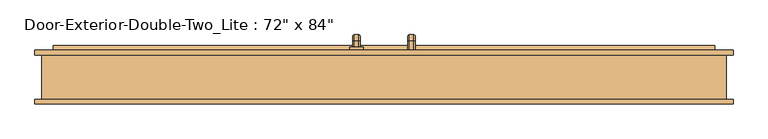
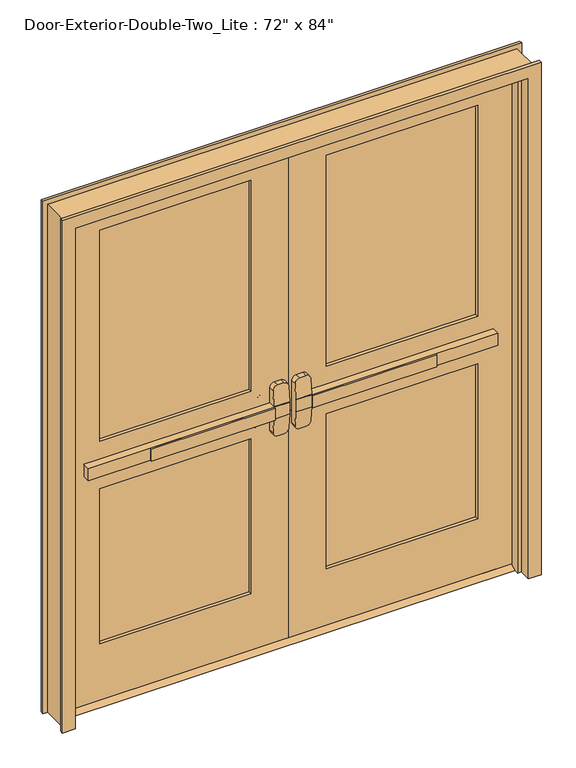
"""IFC4 building model written with IfcOpenShell, lengths in millimetres: door geometry."""

from ifc_helpers import new_model, si_unit, point, frame, frame_2d, origin, place, context, project, spatial, polyline, circle_curve, ellipse_curve, trimmed, segment, composite_curve, outline, extrude, faceted_brep, source, transform, mapped, element, save
from ifc_brep_helpers import plane_surface, cylinder_surface, revolved_surface, advanced_brep


def door_1ff579ad(model_context):
    return source(origin(), model_context, "Body", "SolidModel", [
        extrude(outline(polyline([(-575.7333333, -14.2875), (-575.7333333, -7.9375), (-76.2, -7.9375), (-76.2, -14.2875), (-575.7333333, -14.2875)])), frame((0.0, 0.0, 990.6), z_axis=(0.0, 0.0, 1.0), x_axis=(1.0, 0.0, 0.0)), (0.0, 0.0, 1.0), 50.8),
        advanced_brep(
        [(-12.7, -7.9375, 1041.4), (-76.2, -7.9375, 1041.4), (-825.5, -7.9375, 1041.4), (-825.5, -7.9375, 990.6), (-76.2, -7.9375, 990.6), (-12.7, -7.9375, 990.6), (-825.5, 23.8125, 1041.4), (-76.2, 23.8125, 1041.4), (-76.2, 23.8125, 1104.9), (-57.15, 23.8125, 1123.95), (-31.75, 23.8125, 1123.95), (-12.7, 23.8125, 1104.9), (-12.7, 23.8125, 927.1), (-31.75, 23.8125, 908.05), (-57.15, 23.8125, 908.05), (-76.2, 23.8125, 927.1), (-76.2, 23.8125, 990.6), (-825.5, 23.8125, 990.6), (-12.7, -4.7622533, 1041.4), (-76.2, -4.7622533, 1041.4), (-12.7, -4.7622533, 990.6), (-12.7, 0.2479269, 927.1), (-12.7, 0.2479269, 1104.9), (-76.2, -4.7622533, 990.6), (-76.2, 0.2479269, 1104.9), (-76.2, 0.2479269, 927.1), (-57.15, 1.750981, 1123.95), (-31.75, 1.750981, 1123.95), (-31.75, 1.750981, 908.05), (-57.15, 1.750981, 908.05)],
        [
            (0, 1),
            (1, 2),
            (2, 3),
            (3, 4),
            (4, 5),
            (5, 0),
            (6, 7),
            (7, 8),
            (8, 9, circle_curve(frame((-57.15, 23.8125, 1104.9), z_axis=(0.0, 1.0, 0.0), x_axis=(-1.0, 0.0, 0.0)), 19.05)),
            (9, 10),
            (10, 11, circle_curve(frame((-31.75, 23.8125, 1104.9), z_axis=(0.0, 1.0, 0.0), x_axis=(-1.0, 0.0, 0.0)), 19.05)),
            (11, 12),
            (12, 13, circle_curve(frame((-31.75, 23.8125, 927.1), z_axis=(0.0, 1.0, 0.0), x_axis=(-1.0, 0.0, 0.0)), 19.05)),
            (13, 14),
            (14, 15, circle_curve(frame((-57.15, 23.8125, 927.1), z_axis=(0.0, 1.0, 0.0), x_axis=(-1.0, 0.0, 0.0)), 19.05)),
            (15, 16),
            (16, 17),
            (17, 6),
            (0, 18),
            (18, 19),
            (19, 7),
            (6, 2),
            (5, 20),
            (20, 21),
            (21, 12),
            (11, 22),
            (22, 18),
            (16, 23),
            (23, 20),
            (3, 17),
            (19, 24),
            (24, 8),
            (15, 25),
            (25, 23),
            (9, 26),
            (26, 27),
            (27, 10),
            (13, 28),
            (28, 29),
            (29, 14),
            (29, 25, ellipse_curve(frame((-57.15, 0.2479269, 927.1), z_axis=(0.0, 0.9969018152893365, 0.07865602756830282), x_axis=(0.0, -0.07865602756830208, 0.9969018152893365)), 19.1092038, 19.05)),
            (24, 26, ellipse_curve(frame((-57.15, 0.2479269, 1104.9), z_axis=(0.0, 0.9969018152893376, -0.07865602756828934), x_axis=(0.0, -0.078656027568288, -0.9969018152893377)), 19.1092038, 19.05)),
            (27, 22, ellipse_curve(frame((-31.75, 0.2479269, 1104.9), z_axis=(0.0, 0.9969018152893376, -0.07865602756828934), x_axis=(0.0, -0.078656027568288, -0.9969018152893377)), 19.1092038, 19.05)),
            (21, 28, ellipse_curve(frame((-31.75, 0.2479269, 927.1), z_axis=(0.0, 0.9969018152893365, 0.07865602756830282), x_axis=(0.0, -0.07865602756830208, 0.9969018152893365)), 19.1092038, 19.05)),
        ],
        [
            plane_surface(frame((-12.7, -7.9375, 1041.4), z_axis=(0.0, -1.0, 0.0), x_axis=(1.0, 0.0, 0.0))),
            plane_surface(frame((-12.7, 23.8125, 1041.4), z_axis=(0.0, 1.0, 0.0), x_axis=(-1.0, 0.0, 0.0))),
            plane_surface(frame((-825.5, -7.9375, 1041.4), z_axis=(0.0, 0.0, 1.0), x_axis=(0.0, 1.0, 0.0))),
            plane_surface(frame((-12.7, -7.9375, 1041.4), z_axis=(1.0, 0.0, 0.0), x_axis=(0.0, 1.0, 0.0))),
            plane_surface(frame((-12.7, -7.9375, 990.6), z_axis=(0.0, 0.0, -1.0), x_axis=(0.0, 1.0, 0.0))),
            plane_surface(frame((-825.5, -7.9375, 990.6), z_axis=(-1.0, 0.0, 0.0), x_axis=(0.0, 1.0, 0.0))),
            plane_surface(frame((-76.2, -4.7622533, 927.1), z_axis=(-1.0, 0.0, 0.0), x_axis=(0.0, 1.0, 0.0))),
            plane_surface(frame((-57.15, -4.7622533, 1123.95), z_axis=(0.0, 0.0, 1.0), x_axis=(0.0, 1.0, 0.0))),
            plane_surface(frame((-31.75, -4.7622533, 908.05), z_axis=(0.0, 0.0, -1.0), x_axis=(0.0, 1.0, 0.0))),
            cylinder_surface(frame((-57.15, 23.8125, 927.1), z_axis=(0.0, -1.0, 0.0), x_axis=(-1.0, 0.0, 0.0)), 19.05),
            cylinder_surface(frame((-57.15, 23.8125, 1104.9), z_axis=(0.0, -1.0, 0.0), x_axis=(-1.0, 0.0, 0.0)), 19.05),
            cylinder_surface(frame((-31.75, 23.8125, 1104.9), z_axis=(0.0, -1.0, 0.0), x_axis=(-1.0, 0.0, 0.0)), 19.05),
            cylinder_surface(frame((-31.75, 23.8125, 927.1), z_axis=(0.0, -1.0, 0.0), x_axis=(-1.0, 0.0, 0.0)), 19.05),
            plane_surface(frame((-76.2, -4.7622533, 1041.4), z_axis=(0.0, -0.9969018152893376, 0.07865602756828934), x_axis=(1.0, 0.0, 0.0))),
            plane_surface(frame((-76.2, 1.750981, 908.05), z_axis=(0.0, -0.9969018152893365, -0.07865602756830282), x_axis=(1.0, 0.0, 0.0))),
        ],
        [
            (0, [[1, 2, 3, 4, 5, 6]]),
            (1, [[7, 8, 9, 10, 11, 12, 13, 14, 15, 16, 17, 18]]),
            (2, [[-2, -1, 19, 20, 21, -7, 22]]),
            (3, [[23, 24, 25, -12, 26, 27, -19, -6]]),
            (4, [[-17, 28, 29, -23, -5, -4, 30]]),
            (5, [[-22, -18, -30, -3]]),
            (6, [[-21, 31, 32, -8]]),
            (6, [[33, 34, -28, -16]]),
            (7, [[35, 36, 37, -10]]),
            (8, [[38, 39, 40, -14]]),
            (9, [[-40, 41, -33, -15]]),
            (10, [[-32, 42, -35, -9]]),
            (11, [[-37, 43, -26, -11]]),
            (12, [[-25, 44, -38, -13]]),
            (13, [[-27, -43, -36, -42, -31, -20]]),
            (14, [[-29, -34, -41, -39, -44, -24]]),
        ],
    ),
        extrude(outline(polyline([(68.2625, 12.7), (93.6625, 0.0), (-1.5875, 0.0), (23.8125, 12.7), (68.2625, 12.7)])), frame((-914.4, 0.0, 0.0), z_axis=(1.0, 0.0, 0.0), x_axis=(0.0, 1.0, 0.0)), (0.0, 0.0, 1.0), 1828.8),
        extrude(outline(polyline([(575.7333333, -14.2875), (76.2, -14.2875), (76.2, -7.9375), (575.7333333, -7.9375), (575.7333333, -14.2875)])), frame((0.0, 0.0, 990.6), z_axis=(0.0, 0.0, 1.0), x_axis=(1.0, 0.0, 0.0)), (0.0, 0.0, 1.0), 50.8),
        advanced_brep(
        [(12.7, -7.9375, 1041.4), (12.7, -7.9375, 990.6), (76.2, -7.9375, 990.6), (825.5, -7.9375, 990.6), (825.5, -7.9375, 1041.4), (76.2, -7.9375, 1041.4), (825.5, 23.8125, 1041.4), (825.5, 23.8125, 990.6), (76.2, 23.8125, 990.6), (76.2, 23.8125, 927.1), (57.15, 23.8125, 908.05), (31.75, 23.8125, 908.05), (12.7, 23.8125, 927.1), (12.7, 23.8125, 1104.9), (31.75, 23.8125, 1123.95), (57.15, 23.8125, 1123.95), (76.2, 23.8125, 1104.9), (76.2, 23.8125, 1041.4), (76.2, -4.7622533, 1041.4), (12.7, -4.7622533, 1041.4), (12.7, 0.2479269, 1104.9), (12.7, 0.2479269, 927.1), (12.7, -4.7622533, 990.6), (76.2, -4.7622533, 990.6), (76.2, 0.2479269, 927.1), (76.2, 0.2479269, 1104.9), (31.75, 1.750981, 1123.95), (57.15, 1.750981, 1123.95), (57.15, 1.750981, 908.05), (31.75, 1.750981, 908.05)],
        [
            (0, 1),
            (1, 2),
            (2, 3),
            (3, 4),
            (4, 5),
            (5, 0),
            (6, 7),
            (7, 8),
            (8, 9),
            (9, 10, circle_curve(frame((57.15, 23.8125, 927.1), z_axis=(0.0, 1.0, 0.0), x_axis=(1.0, 0.0, 0.0)), 19.05)),
            (10, 11),
            (11, 12, circle_curve(frame((31.75, 23.8125, 927.1), z_axis=(0.0, 1.0, 0.0), x_axis=(1.0, 0.0, 0.0)), 19.05)),
            (12, 13),
            (13, 14, circle_curve(frame((31.75, 23.8125, 1104.9), z_axis=(0.0, 1.0, 0.0), x_axis=(1.0, 0.0, 0.0)), 19.05)),
            (14, 15),
            (15, 16, circle_curve(frame((57.15, 23.8125, 1104.9), z_axis=(0.0, 1.0, 0.0), x_axis=(1.0, 0.0, 0.0)), 19.05)),
            (16, 17),
            (17, 6),
            (4, 6),
            (17, 18),
            (18, 19),
            (19, 0),
            (19, 20),
            (20, 13),
            (12, 21),
            (21, 22),
            (22, 1),
            (7, 3),
            (22, 23),
            (23, 8),
            (23, 24),
            (24, 9),
            (16, 25),
            (25, 18),
            (14, 26),
            (26, 27),
            (27, 15),
            (10, 28),
            (28, 29),
            (29, 11),
            (24, 28, ellipse_curve(frame((57.15, 0.2479269, 927.1), z_axis=(0.0, 0.9969018152893365, 0.07865602756830282), x_axis=(0.0, -0.07865602756830208, 0.9969018152893365)), 19.1092038, 19.05)),
            (27, 25, ellipse_curve(frame((57.15, 0.2479269, 1104.9), z_axis=(0.0, 0.9969018152893376, -0.07865602756828934), x_axis=(0.0, -0.078656027568288, -0.9969018152893377)), 19.1092038, 19.05)),
            (20, 26, ellipse_curve(frame((31.75, 0.2479269, 1104.9), z_axis=(0.0, 0.9969018152893376, -0.07865602756828934), x_axis=(0.0, -0.078656027568288, -0.9969018152893377)), 19.1092038, 19.05)),
            (29, 21, ellipse_curve(frame((31.75, 0.2479269, 927.1), z_axis=(0.0, 0.9969018152893365, 0.07865602756830282), x_axis=(0.0, -0.07865602756830208, 0.9969018152893365)), 19.1092038, 19.05)),
        ],
        [
            plane_surface(frame((12.7, -7.9375, 1041.4), z_axis=(0.0, -1.0, 0.0), x_axis=(-1.0, 0.0, 0.0))),
            plane_surface(frame((12.7, 23.8125, 1041.4), z_axis=(0.0, 1.0, 0.0), x_axis=(1.0, 0.0, 0.0))),
            plane_surface(frame((825.5, -7.9375, 1041.4), z_axis=(0.0, 0.0, 1.0), x_axis=(0.0, 1.0, 0.0))),
            plane_surface(frame((12.7, -7.9375, 1041.4), z_axis=(-1.0, 0.0, 0.0), x_axis=(0.0, 1.0, 0.0))),
            plane_surface(frame((12.7, -7.9375, 990.6), z_axis=(0.0, 0.0, -1.0), x_axis=(0.0, 1.0, 0.0))),
            plane_surface(frame((825.5, -7.9375, 990.6), z_axis=(1.0, 0.0, 0.0), x_axis=(0.0, 1.0, 0.0))),
            plane_surface(frame((76.2, -4.7622533, 927.1), z_axis=(1.0, 0.0, 0.0), x_axis=(0.0, 1.0, 0.0))),
            plane_surface(frame((57.15, -4.7622533, 1123.95), z_axis=(0.0, 0.0, 1.0), x_axis=(0.0, 1.0, 0.0))),
            plane_surface(frame((31.75, -4.7622533, 908.05), z_axis=(0.0, 0.0, -1.0), x_axis=(0.0, 1.0, 0.0))),
            cylinder_surface(frame((57.15, 23.8125, 927.1), z_axis=(0.0, -1.0, 0.0), x_axis=(1.0, 0.0, 0.0)), 19.05),
            cylinder_surface(frame((57.15, 23.8125, 1104.9), z_axis=(0.0, -1.0, 0.0), x_axis=(1.0, 0.0, 0.0)), 19.05),
            cylinder_surface(frame((31.75, 23.8125, 1104.9), z_axis=(0.0, -1.0, 0.0), x_axis=(1.0, 0.0, 0.0)), 19.05),
            cylinder_surface(frame((31.75, 23.8125, 927.1), z_axis=(0.0, -1.0, 0.0), x_axis=(1.0, 0.0, 0.0)), 19.05),
            plane_surface(frame((76.2, -4.7622533, 1041.4), z_axis=(0.0, -0.9969018152893376, 0.07865602756828934), x_axis=(-1.0, 0.0, 0.0))),
            plane_surface(frame((76.2, 1.750981, 908.05), z_axis=(0.0, -0.9969018152893365, -0.07865602756830282), x_axis=(-1.0, 0.0, 0.0))),
        ],
        [
            (0, [[1, 2, 3, 4, 5, 6]]),
            (1, [[7, 8, 9, 10, 11, 12, 13, 14, 15, 16, 17, 18]]),
            (2, [[19, -18, 20, 21, 22, -6, -5]]),
            (3, [[-1, -22, 23, 24, -13, 25, 26, 27]]),
            (4, [[28, -3, -2, -27, 29, 30, -8]]),
            (5, [[-4, -28, -7, -19]]),
            (6, [[-9, -30, 31, 32]]),
            (6, [[-17, 33, 34, -20]]),
            (7, [[-15, 35, 36, 37]]),
            (8, [[-11, 38, 39, 40]]),
            (9, [[-10, -32, 41, -38]]),
            (10, [[-16, -37, 42, -33]]),
            (11, [[-14, -24, 43, -35]]),
            (12, [[-12, -40, 44, -25]]),
            (13, [[-21, -34, -42, -36, -43, -23]]),
            (14, [[-26, -44, -39, -41, -31, -29]]),
        ],
    ),
        advanced_brep(
        [(66.2, 80.9625, 1017.190625), (66.2, 80.9625, 1014.809375), (69.771875, 80.9625, 1011.2375), (82.6284594, 80.9625, 1011.2375), (86.2, 80.9625, 1014.8090406), (86.2, 80.9625, 1017.190625), (82.628125, 80.9625, 1020.7625), (69.771875, 80.9625, 1020.7625), (66.2, 80.9625, 887.809375), (69.771875, 80.9625, 884.2375), (82.628125, 80.9625, 884.2375), (86.2, 80.9625, 887.809375), (86.2, 80.9625, 890.1909594), (82.6284594, 80.9625, 893.7625), (69.771875, 80.9625, 893.7625), (66.2, 80.9625, 890.190625), (66.2, 106.3625, 1017.190625), (66.2, 120.253125, 1003.3), (66.2, 120.253125, 901.7), (66.2, 106.3625, 887.809375), (66.2, 106.3625, 890.190625), (66.2, 117.871875, 901.7), (66.2, 117.871875, 1003.3), (66.2, 106.3625, 1014.809375), (69.771875, 106.3625, 1011.2375), (82.6284594, 106.3625, 1011.2375), (86.2, 106.3625, 1014.8090406), (86.2, 117.8715406, 1003.3), (86.2, 117.8715406, 901.7), (86.2, 106.3625, 890.1909594), (86.2, 106.3625, 887.809375), (86.2, 120.253125, 901.7), (86.2, 120.253125, 1003.3), (86.2, 106.3625, 1017.190625), (82.628125, 106.3625, 1020.7625), (69.771875, 106.3625, 1020.7625), (69.771875, 114.3, 1003.3), (82.6284594, 114.3, 1003.3), (82.628125, 123.825, 1003.3), (69.771875, 123.825, 1003.3), (69.771875, 114.3, 901.7), (82.6284594, 114.3, 901.7), (82.628125, 123.825, 901.7), (69.771875, 123.825, 901.7), (69.771875, 106.3625, 893.7625), (82.6284594, 106.3625, 893.7625), (82.628125, 106.3625, 884.2375), (69.771875, 106.3625, 884.2375)],
        [
            (0, 1),
            (1, 2, circle_curve(frame((69.771875, 80.9625, 1014.809375), z_axis=(0.0, -1.0, 0.0), x_axis=(0.0, 0.0, 1.0)), 3.571875)),
            (2, 3),
            (3, 4, circle_curve(frame((82.6284594, 80.9625, 1014.8090406), z_axis=(0.0, -1.0, 0.0), x_axis=(0.0, 0.0, 1.0)), 3.5715406)),
            (4, 5),
            (5, 6, circle_curve(frame((82.628125, 80.9625, 1017.190625), z_axis=(0.0, -1.0, 0.0), x_axis=(0.0, 0.0, 1.0)), 3.571875)),
            (6, 7),
            (7, 0, circle_curve(frame((69.771875, 80.9625, 1017.190625), z_axis=(0.0, -1.0, 0.0), x_axis=(0.0, 0.0, 1.0)), 3.571875)),
            (8, 9, circle_curve(frame((69.771875, 80.9625, 887.809375), z_axis=(0.0, -1.0, 0.0), x_axis=(0.0, 0.0, -1.0)), 3.571875)),
            (9, 10),
            (10, 11, circle_curve(frame((82.628125, 80.9625, 887.809375), z_axis=(0.0, -1.0, 0.0), x_axis=(0.0, 0.0, -1.0)), 3.571875)),
            (11, 12),
            (12, 13, circle_curve(frame((82.6284594, 80.9625, 890.1909594), z_axis=(0.0, -1.0, 0.0), x_axis=(0.0, 0.0, -1.0)), 3.5715406)),
            (13, 14),
            (14, 15, circle_curve(frame((69.771875, 80.9625, 890.190625), z_axis=(0.0, -1.0, 0.0), x_axis=(0.0, 0.0, -1.0)), 3.571875)),
            (15, 8),
            (0, 16),
            (16, 17, circle_curve(frame((66.2, 106.3625, 1003.3), z_axis=(-1.0, 0.0, 0.0), x_axis=(0.0, 0.0, 1.0)), 13.890625)),
            (17, 18),
            (18, 19, circle_curve(frame((66.2, 106.3625, 901.7), z_axis=(-1.0, 0.0, 0.0), x_axis=(0.0, 1.0, 0.0)), 13.890625)),
            (19, 8),
            (15, 20),
            (20, 21, circle_curve(frame((66.2, 106.3625, 901.7), z_axis=(1.0, 0.0, 0.0), x_axis=(0.0, 1.0, 0.0)), 11.509375)),
            (21, 22),
            (22, 23, circle_curve(frame((66.2, 106.3625, 1003.3), z_axis=(1.0, 0.0, 0.0), x_axis=(0.0, 0.0, 1.0)), 11.509375)),
            (23, 1),
            (23, 24, circle_curve(frame((69.771875, 106.3625, 1014.809375), z_axis=(0.0, -1.0, 0.0), x_axis=(0.0, 0.0, 1.0)), 3.571875)),
            (24, 2),
            (24, 25),
            (25, 3),
            (25, 26, circle_curve(frame((82.6284594, 106.3625, 1014.8090406), z_axis=(0.0, -1.0, 0.0), x_axis=(0.0, 0.0, 1.0)), 3.5715406)),
            (26, 4),
            (26, 27, circle_curve(frame((86.2, 106.3625, 1003.3), z_axis=(-1.0, 0.0, 0.0), x_axis=(0.0, 0.0, 1.0)), 11.5090406)),
            (27, 28),
            (28, 29, circle_curve(frame((86.2, 106.3625, 901.7), z_axis=(-1.0, 0.0, 0.0), x_axis=(0.0, 1.0, 0.0)), 11.5090406)),
            (29, 12),
            (11, 30),
            (30, 31, circle_curve(frame((86.2, 106.3625, 901.7), z_axis=(1.0, 0.0, 0.0), x_axis=(0.0, 1.0, 0.0)), 13.890625)),
            (31, 32),
            (32, 33, circle_curve(frame((86.2, 106.3625, 1003.3), z_axis=(1.0, 0.0, 0.0), x_axis=(0.0, 0.0, 1.0)), 13.890625)),
            (33, 5),
            (33, 34, circle_curve(frame((82.628125, 106.3625, 1017.190625), z_axis=(0.0, -1.0, 0.0), x_axis=(0.0, 0.0, 1.0)), 3.571875)),
            (34, 6),
            (34, 35),
            (35, 7),
            (35, 16, circle_curve(frame((69.771875, 106.3625, 1017.190625), z_axis=(0.0, -1.0, 0.0), x_axis=(0.0, 0.0, 1.0)), 3.571875)),
            (36, 24, circle_curve(frame((69.771875, 106.3625, 1003.3), z_axis=(1.0, 0.0, 0.0), x_axis=(0.0, 0.0, 1.0)), 7.9375)),
            (22, 36, circle_curve(frame((69.771875, 117.871875, 1003.3), z_axis=(0.0, 0.0, 1.0), x_axis=(0.0, 1.0, 0.0)), 3.571875)),
            (37, 25, circle_curve(frame((82.6284594, 106.3625, 1003.3), z_axis=(1.0, 0.0, 0.0), x_axis=(0.0, 0.0, 1.0)), 7.9375)),
            (36, 37),
            (37, 27, circle_curve(frame((82.6284594, 117.8715406, 1003.3), z_axis=(0.0, 0.0, 1.0), x_axis=(0.0, 1.0, 0.0)), 3.5715406)),
            (38, 34, circle_curve(frame((82.628125, 106.3625, 1003.3), z_axis=(1.0, 0.0, 0.0), x_axis=(0.0, 0.0, 1.0)), 17.4625)),
            (32, 38, circle_curve(frame((82.628125, 120.253125, 1003.3), z_axis=(0.0, 0.0, 1.0), x_axis=(0.0, 1.0, 0.0)), 3.571875)),
            (39, 35, circle_curve(frame((69.771875, 106.3625, 1003.3), z_axis=(1.0, 0.0, 0.0), x_axis=(0.0, 0.0, 1.0)), 17.4625)),
            (38, 39),
            (39, 17, circle_curve(frame((69.771875, 120.253125, 1003.3), z_axis=(0.0, 0.0, 1.0), x_axis=(0.0, 1.0, 0.0)), 3.571875)),
            (21, 40, circle_curve(frame((69.771875, 117.871875, 901.7), z_axis=(0.0, 0.0, 1.0), x_axis=(0.0, 1.0, 0.0)), 3.571875)),
            (40, 36),
            (40, 41),
            (41, 37),
            (41, 28, circle_curve(frame((82.6284594, 117.8715406, 901.7), z_axis=(0.0, 0.0, 1.0), x_axis=(0.0, 1.0, 0.0)), 3.5715406)),
            (31, 42, circle_curve(frame((82.628125, 120.253125, 901.7), z_axis=(0.0, 0.0, 1.0), x_axis=(0.0, 1.0, 0.0)), 3.571875)),
            (42, 38),
            (42, 43),
            (43, 39),
            (43, 18, circle_curve(frame((69.771875, 120.253125, 901.7), z_axis=(0.0, 0.0, 1.0), x_axis=(0.0, 1.0, 0.0)), 3.571875)),
            (44, 40, circle_curve(frame((69.771875, 106.3625, 901.7), z_axis=(1.0, 0.0, 0.0), x_axis=(0.0, 1.0, 0.0)), 7.9375)),
            (20, 44, circle_curve(frame((69.771875, 106.3625, 890.190625), z_axis=(0.0, 1.0, 0.0), x_axis=(0.0, 0.0, -1.0)), 3.571875)),
            (45, 41, circle_curve(frame((82.6284594, 106.3625, 901.7), z_axis=(1.0, 0.0, 0.0), x_axis=(0.0, 1.0, 0.0)), 7.9375)),
            (44, 45),
            (45, 29, circle_curve(frame((82.6284594, 106.3625, 890.1909594), z_axis=(0.0, 1.0, 0.0), x_axis=(0.0, 0.0, -1.0)), 3.5715406)),
            (46, 42, circle_curve(frame((82.628125, 106.3625, 901.7), z_axis=(1.0, 0.0, 0.0), x_axis=(0.0, 1.0, 0.0)), 17.4625)),
            (30, 46, circle_curve(frame((82.628125, 106.3625, 887.809375), z_axis=(0.0, 1.0, 0.0), x_axis=(0.0, 0.0, -1.0)), 3.571875)),
            (47, 43, circle_curve(frame((69.771875, 106.3625, 901.7), z_axis=(1.0, 0.0, 0.0), x_axis=(0.0, 1.0, 0.0)), 17.4625)),
            (46, 47),
            (47, 19, circle_curve(frame((69.771875, 106.3625, 887.809375), z_axis=(0.0, 1.0, 0.0), x_axis=(0.0, 0.0, -1.0)), 3.571875)),
            (14, 44),
            (13, 45),
            (10, 46),
            (9, 47),
        ],
        [
            plane_surface(frame((76.2, 80.9625, 1016.0), z_axis=(0.0, -1.0, 0.0), x_axis=(1.0, 0.0, 0.0))),
            plane_surface(frame((76.2, 80.9625, 889.0), z_axis=(0.0, -1.0, 0.0), x_axis=(1.0, 0.0, 0.0))),
            plane_surface(frame((66.2, 80.9625, 1017.190625), z_axis=(-1.0, 0.0, 0.0), x_axis=(0.0, 1.0, 0.0))),
            cylinder_surface(frame((69.771875, 80.9625, 1014.809375), z_axis=(0.0, -1.0, 0.0), x_axis=(0.0, 0.0, 1.0)), 3.571875),
            plane_surface(frame((69.771875, 80.9625, 1011.2375), z_axis=(0.0, 0.0, -1.0), x_axis=(0.0, 1.0, 0.0))),
            cylinder_surface(frame((82.6284594, 80.9625, 1014.8090406), z_axis=(0.0, -1.0, 0.0), x_axis=(0.0, 0.0, 1.0)), 3.5715406),
            plane_surface(frame((86.2, 80.9625, 1014.8090406), z_axis=(1.0, 0.0, 0.0), x_axis=(0.0, 1.0, 0.0))),
            cylinder_surface(frame((82.628125, 80.9625, 1017.190625), z_axis=(0.0, -1.0, 0.0), x_axis=(0.0, 0.0, 1.0)), 3.571875),
            plane_surface(frame((82.628125, 80.9625, 1020.7625), z_axis=(0.0, 0.0, 1.0), x_axis=(0.0, 1.0, 0.0))),
            cylinder_surface(frame((69.771875, 80.9625, 1017.190625), z_axis=(0.0, -1.0, 0.0), x_axis=(0.0, 0.0, 1.0)), 3.571875),
            revolved_surface(trimmed(ellipse_curve(frame((69.771875, 106.3625, 1014.809375), z_axis=(0.0, -1.0, 0.0), x_axis=(0.0, 0.0, 1.0)), 3.571875, 3.571875), [point((66.2, 106.3625, 1014.809375))], [point((69.771875, 106.3625, 1011.2375))], True, "CARTESIAN"), (76.2, 106.3625, 1003.3), (-1.0, 0.0, 0.0)),
            revolved_surface(polyline([(69.771875, 106.3625, 1011.2375), (82.6284594, 106.3625, 1011.2375)]), (76.2, 106.3625, 1003.3), (-1.0, 0.0, 0.0)),
            revolved_surface(trimmed(ellipse_curve(frame((82.6284594, 106.3625, 1014.8090406), z_axis=(0.0, -1.0, 0.0), x_axis=(0.0, 0.0, 1.0)), 3.5715406, 3.5715406), [point((82.6284594, 106.3625, 1011.2375))], [point((86.2, 106.3625, 1014.8090406))], True, "CARTESIAN"), (76.2, 106.3625, 1003.3), (-1.0, 0.0, 0.0)),
            revolved_surface(trimmed(ellipse_curve(frame((82.628125, 106.3625, 1017.190625), z_axis=(0.0, -1.0, 0.0), x_axis=(0.0, 0.0, 1.0)), 3.571875, 3.571875), [point((86.2, 106.3625, 1017.190625))], [point((82.628125, 106.3625, 1020.7625))], True, "CARTESIAN"), (76.2, 106.3625, 1003.3), (-1.0, 0.0, 0.0)),
            cylinder_surface(frame((76.2, 106.3625, 1003.3), z_axis=(-1.0, 0.0, 0.0), x_axis=(0.0, 0.0, 1.0)), 17.4625),
            revolved_surface(trimmed(ellipse_curve(frame((69.771875, 106.3625, 1017.190625), z_axis=(0.0, -1.0, 0.0), x_axis=(0.0, 0.0, 1.0)), 3.571875, 3.571875), [point((69.771875, 106.3625, 1020.7625))], [point((66.2, 106.3625, 1017.190625))], True, "CARTESIAN"), (76.2, 106.3625, 1003.3), (-1.0, 0.0, 0.0)),
            cylinder_surface(frame((69.771875, 117.871875, 1003.3), z_axis=(0.0, 0.0, 1.0), x_axis=(0.0, 1.0, 0.0)), 3.571875),
            plane_surface(frame((69.771875, 114.3, 1003.3), z_axis=(0.0, -1.0, 0.0), x_axis=(0.0, 0.0, -1.0))),
            cylinder_surface(frame((82.6284594, 117.8715406, 1003.3), z_axis=(0.0, 0.0, 1.0), x_axis=(0.0, 1.0, 0.0)), 3.5715406),
            cylinder_surface(frame((82.628125, 120.253125, 1003.3), z_axis=(0.0, 0.0, 1.0), x_axis=(0.0, 1.0, 0.0)), 3.571875),
            plane_surface(frame((82.628125, 123.825, 1003.3), z_axis=(0.0, 1.0, 0.0), x_axis=(0.0, 0.0, -1.0))),
            cylinder_surface(frame((69.771875, 120.253125, 1003.3), z_axis=(0.0, 0.0, 1.0), x_axis=(0.0, 1.0, 0.0)), 3.571875),
            revolved_surface(trimmed(ellipse_curve(frame((69.771875, 117.871875, 901.7), z_axis=(0.0, 0.0, 1.0), x_axis=(0.0, 1.0, 0.0)), 3.571875, 3.571875), [point((66.2, 117.871875, 901.7))], [point((69.771875, 114.3, 901.7))], True, "CARTESIAN"), (76.2, 106.3625, 901.7), (-1.0, 0.0, 0.0)),
            revolved_surface(polyline([(69.771875, 114.3, 901.7), (82.6284594, 114.3, 901.7)]), (76.2, 106.3625, 901.7), (-1.0, 0.0, 0.0)),
            revolved_surface(trimmed(ellipse_curve(frame((82.6284594, 117.8715406, 901.7), z_axis=(0.0, 0.0, 1.0), x_axis=(0.0, 1.0, 0.0)), 3.5715406, 3.5715406), [point((82.6284594, 114.3, 901.7))], [point((86.2, 117.8715406, 901.7))], True, "CARTESIAN"), (76.2, 106.3625, 901.7), (-1.0, 0.0, 0.0)),
            revolved_surface(trimmed(ellipse_curve(frame((82.628125, 120.253125, 901.7), z_axis=(0.0, 0.0, 1.0), x_axis=(0.0, 1.0, 0.0)), 3.571875, 3.571875), [point((86.2, 120.253125, 901.7))], [point((82.628125, 123.825, 901.7))], True, "CARTESIAN"), (76.2, 106.3625, 901.7), (-1.0, 0.0, 0.0)),
            cylinder_surface(frame((76.2, 106.3625, 901.7), z_axis=(-1.0, 0.0, 0.0), x_axis=(0.0, 1.0, 0.0)), 17.4625),
            revolved_surface(trimmed(ellipse_curve(frame((69.771875, 120.253125, 901.7), z_axis=(0.0, 0.0, 1.0), x_axis=(0.0, 1.0, 0.0)), 3.571875, 3.571875), [point((69.771875, 123.825, 901.7))], [point((66.2, 120.253125, 901.7))], True, "CARTESIAN"), (76.2, 106.3625, 901.7), (-1.0, 0.0, 0.0)),
            cylinder_surface(frame((69.771875, 106.3625, 890.190625), z_axis=(0.0, 1.0, 0.0), x_axis=(0.0, 0.0, -1.0)), 3.571875),
            plane_surface(frame((69.771875, 106.3625, 893.7625), z_axis=(0.0, 0.0, 1.0), x_axis=(0.0, -1.0, 0.0))),
            cylinder_surface(frame((82.6284594, 106.3625, 890.1909594), z_axis=(0.0, 1.0, 0.0), x_axis=(0.0, 0.0, -1.0)), 3.5715406),
            cylinder_surface(frame((82.628125, 106.3625, 887.809375), z_axis=(0.0, 1.0, 0.0), x_axis=(0.0, 0.0, -1.0)), 3.571875),
            plane_surface(frame((82.628125, 106.3625, 884.2375), z_axis=(0.0, 0.0, -1.0), x_axis=(0.0, -1.0, 0.0))),
            cylinder_surface(frame((69.771875, 106.3625, 887.809375), z_axis=(0.0, 1.0, 0.0), x_axis=(0.0, 0.0, -1.0)), 3.571875),
        ],
        [
            (0, [[1, 2, 3, 4, 5, 6, 7, 8]]),
            (1, [[9, 10, 11, 12, 13, 14, 15, 16]]),
            (2, [[-1, 17, 18, 19, 20, 21, -16, 22, 23, 24, 25, 26]]),
            (3, [[-2, -26, 27, 28]]),
            (4, [[-3, -28, 29, 30]]),
            (5, [[-4, -30, 31, 32]]),
            (6, [[-5, -32, 33, 34, 35, 36, -12, 37, 38, 39, 40, 41]]),
            (7, [[-6, -41, 42, 43]]),
            (8, [[-7, -43, 44, 45]]),
            (9, [[-8, -45, 46, -17]]),
            (10, [[47, -27, -25, 48]]),
            (11, [[49, -29, -47, 50]]),
            (12, [[-33, -31, -49, 51]]),
            (13, [[52, -42, -40, 53]]),
            (14, [[54, -44, -52, 55]]),
            (15, [[-18, -46, -54, 56]]),
            (16, [[-48, -24, 57, 58]]),
            (17, [[-50, -58, 59, 60]]),
            (18, [[-51, -60, 61, -34]]),
            (19, [[-53, -39, 62, 63]]),
            (20, [[-55, -63, 64, 65]]),
            (21, [[-56, -65, 66, -19]]),
            (22, [[67, -57, -23, 68]]),
            (23, [[69, -59, -67, 70]]),
            (24, [[-35, -61, -69, 71]]),
            (25, [[72, -62, -38, 73]]),
            (26, [[74, -64, -72, 75]]),
            (27, [[-20, -66, -74, 76]]),
            (28, [[-68, -22, -15, 77]]),
            (29, [[-70, -77, -14, 78]]),
            (30, [[-71, -78, -13, -36]]),
            (31, [[-73, -37, -11, 79]]),
            (32, [[-75, -79, -10, 80]]),
            (33, [[-76, -80, -9, -21]]),
        ],
    ),
        extrude(outline(composite_curve([segment(trimmed(circle_curve(frame_2d((1113.0338574, 76.2)), 89.3016225), [point((1193.8, 114.3))], [point((1193.8, 38.1))], False, "CARTESIAN"), True, "CONTINUOUS"), segment(polyline([(1193.8, 38.1), (838.2, 38.1)]), True, "CONTINUOUS"), segment(trimmed(circle_curve(frame_2d((918.9661426, 76.2)), 89.3016225), [point((838.2, 38.1))], [point((838.2, 114.3))], False, "CARTESIAN"), True, "CONTINUOUS"), segment(polyline([(838.2, 114.3), (1193.8, 114.3)]), True, "CONTINUOUS")], self_intersect=False)), frame((0.0, 68.2625, 0.0), z_axis=(0.0, 1.0, 0.0), x_axis=(0.0, 0.0, 1.0)), (0.0, 0.0, 1.0), 12.7),
        advanced_brep(
        [(-86.2, 80.9625, 1017.190625), (-86.2, 80.9625, 1014.809375), (-82.628125, 80.9625, 1011.2375), (-69.7715406, 80.9625, 1011.2375), (-66.2, 80.9625, 1014.8090406), (-66.2, 80.9625, 1017.190625), (-69.771875, 80.9625, 1020.7625), (-82.628125, 80.9625, 1020.7625), (-86.2, 80.9625, 887.809375), (-82.628125, 80.9625, 884.2375), (-69.771875, 80.9625, 884.2375), (-66.2, 80.9625, 887.809375), (-66.2, 80.9625, 890.1909594), (-69.7715406, 80.9625, 893.7625), (-82.628125, 80.9625, 893.7625), (-86.2, 80.9625, 890.190625), (-86.2, 106.3625, 1017.190625), (-86.2, 120.253125, 1003.3), (-86.2, 120.253125, 901.7), (-86.2, 106.3625, 887.809375), (-86.2, 106.3625, 890.190625), (-86.2, 117.871875, 901.7), (-86.2, 117.871875, 1003.3), (-86.2, 106.3625, 1014.809375), (-82.628125, 106.3625, 1011.2375), (-69.7715406, 106.3625, 1011.2375), (-66.2, 106.3625, 1014.8090406), (-66.2, 117.8715406, 1003.3), (-66.2, 117.8715406, 901.7), (-66.2, 106.3625, 890.1909594), (-66.2, 106.3625, 887.809375), (-66.2, 120.253125, 901.7), (-66.2, 120.253125, 1003.3), (-66.2, 106.3625, 1017.190625), (-69.771875, 106.3625, 1020.7625), (-82.628125, 106.3625, 1020.7625), (-82.628125, 114.3, 1003.3), (-69.7715406, 114.3, 1003.3), (-69.771875, 123.825, 1003.3), (-82.628125, 123.825, 1003.3), (-82.628125, 114.3, 901.7), (-69.7715406, 114.3, 901.7), (-69.771875, 123.825, 901.7), (-82.628125, 123.825, 901.7), (-82.628125, 106.3625, 893.7625), (-69.7715406, 106.3625, 893.7625), (-69.771875, 106.3625, 884.2375), (-82.628125, 106.3625, 884.2375)],
        [
            (0, 1),
            (1, 2, circle_curve(frame((-82.628125, 80.9625, 1014.809375), z_axis=(0.0, -1.0, 0.0), x_axis=(0.0, 0.0, 1.0)), 3.571875)),
            (2, 3),
            (3, 4, circle_curve(frame((-69.7715406, 80.9625, 1014.8090406), z_axis=(0.0, -1.0, 0.0), x_axis=(0.0, 0.0, 1.0)), 3.5715406)),
            (4, 5),
            (5, 6, circle_curve(frame((-69.771875, 80.9625, 1017.190625), z_axis=(0.0, -1.0, 0.0), x_axis=(0.0, 0.0, 1.0)), 3.571875)),
            (6, 7),
            (7, 0, circle_curve(frame((-82.628125, 80.9625, 1017.190625), z_axis=(0.0, -1.0, 0.0), x_axis=(0.0, 0.0, 1.0)), 3.571875)),
            (8, 9, circle_curve(frame((-82.628125, 80.9625, 887.809375), z_axis=(0.0, -1.0, 0.0), x_axis=(0.0, 0.0, -1.0)), 3.571875)),
            (9, 10),
            (10, 11, circle_curve(frame((-69.771875, 80.9625, 887.809375), z_axis=(0.0, -1.0, 0.0), x_axis=(0.0, 0.0, -1.0)), 3.571875)),
            (11, 12),
            (12, 13, circle_curve(frame((-69.7715406, 80.9625, 890.1909594), z_axis=(0.0, -1.0, 0.0), x_axis=(0.0, 0.0, -1.0)), 3.5715406)),
            (13, 14),
            (14, 15, circle_curve(frame((-82.628125, 80.9625, 890.190625), z_axis=(0.0, -1.0, 0.0), x_axis=(0.0, 0.0, -1.0)), 3.571875)),
            (15, 8),
            (0, 16),
            (16, 17, circle_curve(frame((-86.2, 106.3625, 1003.3), z_axis=(-1.0, 0.0, 0.0), x_axis=(0.0, 0.0, 1.0)), 13.890625)),
            (17, 18),
            (18, 19, circle_curve(frame((-86.2, 106.3625, 901.7), z_axis=(-1.0, 0.0, 0.0), x_axis=(0.0, 1.0, 0.0)), 13.890625)),
            (19, 8),
            (15, 20),
            (20, 21, circle_curve(frame((-86.2, 106.3625, 901.7), z_axis=(1.0, 0.0, 0.0), x_axis=(0.0, 1.0, 0.0)), 11.509375)),
            (21, 22),
            (22, 23, circle_curve(frame((-86.2, 106.3625, 1003.3), z_axis=(1.0, 0.0, 0.0), x_axis=(0.0, 0.0, 1.0)), 11.509375)),
            (23, 1),
            (23, 24, circle_curve(frame((-82.628125, 106.3625, 1014.809375), z_axis=(0.0, -1.0, 0.0), x_axis=(0.0, 0.0, 1.0)), 3.571875)),
            (24, 2),
            (24, 25),
            (25, 3),
            (25, 26, circle_curve(frame((-69.7715406, 106.3625, 1014.8090406), z_axis=(0.0, -1.0, 0.0), x_axis=(0.0, 0.0, 1.0)), 3.5715406)),
            (26, 4),
            (26, 27, circle_curve(frame((-66.2, 106.3625, 1003.3), z_axis=(-1.0, 0.0, 0.0), x_axis=(0.0, 0.0, 1.0)), 11.5090406)),
            (27, 28),
            (28, 29, circle_curve(frame((-66.2, 106.3625, 901.7), z_axis=(-1.0, 0.0, 0.0), x_axis=(0.0, 1.0, 0.0)), 11.5090406)),
            (29, 12),
            (11, 30),
            (30, 31, circle_curve(frame((-66.2, 106.3625, 901.7), z_axis=(1.0, 0.0, 0.0), x_axis=(0.0, 1.0, 0.0)), 13.890625)),
            (31, 32),
            (32, 33, circle_curve(frame((-66.2, 106.3625, 1003.3), z_axis=(1.0, 0.0, 0.0), x_axis=(0.0, 0.0, 1.0)), 13.890625)),
            (33, 5),
            (33, 34, circle_curve(frame((-69.771875, 106.3625, 1017.190625), z_axis=(0.0, -1.0, 0.0), x_axis=(0.0, 0.0, 1.0)), 3.571875)),
            (34, 6),
            (34, 35),
            (35, 7),
            (35, 16, circle_curve(frame((-82.628125, 106.3625, 1017.190625), z_axis=(0.0, -1.0, 0.0), x_axis=(0.0, 0.0, 1.0)), 3.571875)),
            (36, 24, circle_curve(frame((-82.628125, 106.3625, 1003.3), z_axis=(1.0, 0.0, 0.0), x_axis=(0.0, 0.0, 1.0)), 7.9375)),
            (22, 36, circle_curve(frame((-82.628125, 117.871875, 1003.3), z_axis=(0.0, 0.0, 1.0), x_axis=(0.0, 1.0, 0.0)), 3.571875)),
            (37, 25, circle_curve(frame((-69.7715406, 106.3625, 1003.3), z_axis=(1.0, 0.0, 0.0), x_axis=(0.0, 0.0, 1.0)), 7.9375)),
            (36, 37),
            (37, 27, circle_curve(frame((-69.7715406, 117.8715406, 1003.3), z_axis=(0.0, 0.0, 1.0), x_axis=(0.0, 1.0, 0.0)), 3.5715406)),
            (38, 34, circle_curve(frame((-69.771875, 106.3625, 1003.3), z_axis=(1.0, 0.0, 0.0), x_axis=(0.0, 0.0, 1.0)), 17.4625)),
            (32, 38, circle_curve(frame((-69.771875, 120.253125, 1003.3), z_axis=(0.0, 0.0, 1.0), x_axis=(0.0, 1.0, 0.0)), 3.571875)),
            (39, 35, circle_curve(frame((-82.628125, 106.3625, 1003.3), z_axis=(1.0, 0.0, 0.0), x_axis=(0.0, 0.0, 1.0)), 17.4625)),
            (38, 39),
            (39, 17, circle_curve(frame((-82.628125, 120.253125, 1003.3), z_axis=(0.0, 0.0, 1.0), x_axis=(0.0, 1.0, 0.0)), 3.571875)),
            (21, 40, circle_curve(frame((-82.628125, 117.871875, 901.7), z_axis=(0.0, 0.0, 1.0), x_axis=(0.0, 1.0, 0.0)), 3.571875)),
            (40, 36),
            (40, 41),
            (41, 37),
            (41, 28, circle_curve(frame((-69.7715406, 117.8715406, 901.7), z_axis=(0.0, 0.0, 1.0), x_axis=(0.0, 1.0, 0.0)), 3.5715406)),
            (31, 42, circle_curve(frame((-69.771875, 120.253125, 901.7), z_axis=(0.0, 0.0, 1.0), x_axis=(0.0, 1.0, 0.0)), 3.571875)),
            (42, 38),
            (42, 43),
            (43, 39),
            (43, 18, circle_curve(frame((-82.628125, 120.253125, 901.7), z_axis=(0.0, 0.0, 1.0), x_axis=(0.0, 1.0, 0.0)), 3.571875)),
            (44, 40, circle_curve(frame((-82.628125, 106.3625, 901.7), z_axis=(1.0, 0.0, 0.0), x_axis=(0.0, 1.0, 0.0)), 7.9375)),
            (20, 44, circle_curve(frame((-82.628125, 106.3625, 890.190625), z_axis=(0.0, 1.0, 0.0), x_axis=(0.0, 0.0, -1.0)), 3.571875)),
            (45, 41, circle_curve(frame((-69.7715406, 106.3625, 901.7), z_axis=(1.0, 0.0, 0.0), x_axis=(0.0, 1.0, 0.0)), 7.9375)),
            (44, 45),
            (45, 29, circle_curve(frame((-69.7715406, 106.3625, 890.1909594), z_axis=(0.0, 1.0, 0.0), x_axis=(0.0, 0.0, -1.0)), 3.5715406)),
            (46, 42, circle_curve(frame((-69.771875, 106.3625, 901.7), z_axis=(1.0, 0.0, 0.0), x_axis=(0.0, 1.0, 0.0)), 17.4625)),
            (30, 46, circle_curve(frame((-69.771875, 106.3625, 887.809375), z_axis=(0.0, 1.0, 0.0), x_axis=(0.0, 0.0, -1.0)), 3.571875)),
            (47, 43, circle_curve(frame((-82.628125, 106.3625, 901.7), z_axis=(1.0, 0.0, 0.0), x_axis=(0.0, 1.0, 0.0)), 17.4625)),
            (46, 47),
            (47, 19, circle_curve(frame((-82.628125, 106.3625, 887.809375), z_axis=(0.0, 1.0, 0.0), x_axis=(0.0, 0.0, -1.0)), 3.571875)),
            (14, 44),
            (13, 45),
            (10, 46),
            (9, 47),
        ],
        [
            plane_surface(frame((-76.2, 80.9625, 1016.0), z_axis=(0.0, -1.0, 0.0), x_axis=(1.0, 0.0, 0.0))),
            plane_surface(frame((-76.2, 80.9625, 889.0), z_axis=(0.0, -1.0, 0.0), x_axis=(1.0, 0.0, 0.0))),
            plane_surface(frame((-86.2, 80.9625, 1017.190625), z_axis=(-1.0, 0.0, 0.0), x_axis=(0.0, 1.0, 0.0))),
            cylinder_surface(frame((-82.628125, 80.9625, 1014.809375), z_axis=(0.0, -1.0, 0.0), x_axis=(0.0, 0.0, 1.0)), 3.571875),
            plane_surface(frame((-82.628125, 80.9625, 1011.2375), z_axis=(0.0, 0.0, -1.0), x_axis=(0.0, 1.0, 0.0))),
            cylinder_surface(frame((-69.7715406, 80.9625, 1014.8090406), z_axis=(0.0, -1.0, 0.0), x_axis=(0.0, 0.0, 1.0)), 3.5715406),
            plane_surface(frame((-66.2, 80.9625, 1014.8090406), z_axis=(1.0, 0.0, 0.0), x_axis=(0.0, 1.0, 0.0))),
            cylinder_surface(frame((-69.771875, 80.9625, 1017.190625), z_axis=(0.0, -1.0, 0.0), x_axis=(0.0, 0.0, 1.0)), 3.571875),
            plane_surface(frame((-69.771875, 80.9625, 1020.7625), z_axis=(0.0, 0.0, 1.0), x_axis=(0.0, 1.0, 0.0))),
            cylinder_surface(frame((-82.628125, 80.9625, 1017.190625), z_axis=(0.0, -1.0, 0.0), x_axis=(0.0, 0.0, 1.0)), 3.571875),
            revolved_surface(trimmed(ellipse_curve(frame((-82.628125, 106.3625, 1014.809375), z_axis=(0.0, -1.0, 0.0), x_axis=(0.0, 0.0, 1.0)), 3.571875, 3.571875), [point((-86.2, 106.3625, 1014.809375))], [point((-82.628125, 106.3625, 1011.2375))], True, "CARTESIAN"), (-76.2, 106.3625, 1003.3), (-1.0, 0.0, 0.0)),
            revolved_surface(polyline([(-82.628125, 106.3625, 1011.2375), (-69.7715406, 106.3625, 1011.2375)]), (-76.2, 106.3625, 1003.3), (-1.0, 0.0, 0.0)),
            revolved_surface(trimmed(ellipse_curve(frame((-69.7715406, 106.3625, 1014.8090406), z_axis=(0.0, -1.0, 0.0), x_axis=(0.0, 0.0, 1.0)), 3.5715406, 3.5715406), [point((-69.7715406, 106.3625, 1011.2375))], [point((-66.2, 106.3625, 1014.8090406))], True, "CARTESIAN"), (-76.2, 106.3625, 1003.3), (-1.0, 0.0, 0.0)),
            revolved_surface(trimmed(ellipse_curve(frame((-69.771875, 106.3625, 1017.190625), z_axis=(0.0, -1.0, 0.0), x_axis=(0.0, 0.0, 1.0)), 3.571875, 3.571875), [point((-66.2, 106.3625, 1017.190625))], [point((-69.771875, 106.3625, 1020.7625))], True, "CARTESIAN"), (-76.2, 106.3625, 1003.3), (-1.0, 0.0, 0.0)),
            cylinder_surface(frame((-76.2, 106.3625, 1003.3), z_axis=(-1.0, 0.0, 0.0), x_axis=(0.0, 0.0, 1.0)), 17.4625),
            revolved_surface(trimmed(ellipse_curve(frame((-82.628125, 106.3625, 1017.190625), z_axis=(0.0, -1.0, 0.0), x_axis=(0.0, 0.0, 1.0)), 3.571875, 3.571875), [point((-82.628125, 106.3625, 1020.7625))], [point((-86.2, 106.3625, 1017.190625))], True, "CARTESIAN"), (-76.2, 106.3625, 1003.3), (-1.0, 0.0, 0.0)),
            cylinder_surface(frame((-82.628125, 117.871875, 1003.3), z_axis=(0.0, 0.0, 1.0), x_axis=(0.0, 1.0, 0.0)), 3.571875),
            plane_surface(frame((-82.628125, 114.3, 1003.3), z_axis=(0.0, -1.0, 0.0), x_axis=(0.0, 0.0, -1.0))),
            cylinder_surface(frame((-69.7715406, 117.8715406, 1003.3), z_axis=(0.0, 0.0, 1.0), x_axis=(0.0, 1.0, 0.0)), 3.5715406),
            cylinder_surface(frame((-69.771875, 120.253125, 1003.3), z_axis=(0.0, 0.0, 1.0), x_axis=(0.0, 1.0, 0.0)), 3.571875),
            plane_surface(frame((-69.771875, 123.825, 1003.3), z_axis=(0.0, 1.0, 0.0), x_axis=(0.0, 0.0, -1.0))),
            cylinder_surface(frame((-82.628125, 120.253125, 1003.3), z_axis=(0.0, 0.0, 1.0), x_axis=(0.0, 1.0, 0.0)), 3.571875),
            revolved_surface(trimmed(ellipse_curve(frame((-82.628125, 117.871875, 901.7), z_axis=(0.0, 0.0, 1.0), x_axis=(0.0, 1.0, 0.0)), 3.571875, 3.571875), [point((-86.2, 117.871875, 901.7))], [point((-82.628125, 114.3, 901.7))], True, "CARTESIAN"), (-76.2, 106.3625, 901.7), (-1.0, 0.0, 0.0)),
            revolved_surface(polyline([(-82.628125, 114.3, 901.7), (-69.7715406, 114.3, 901.7)]), (-76.2, 106.3625, 901.7), (-1.0, 0.0, 0.0)),
            revolved_surface(trimmed(ellipse_curve(frame((-69.7715406, 117.8715406, 901.7), z_axis=(0.0, 0.0, 1.0), x_axis=(0.0, 1.0, 0.0)), 3.5715406, 3.5715406), [point((-69.7715406, 114.3, 901.7))], [point((-66.2, 117.8715406, 901.7))], True, "CARTESIAN"), (-76.2, 106.3625, 901.7), (-1.0, 0.0, 0.0)),
            revolved_surface(trimmed(ellipse_curve(frame((-69.771875, 120.253125, 901.7), z_axis=(0.0, 0.0, 1.0), x_axis=(0.0, 1.0, 0.0)), 3.571875, 3.571875), [point((-66.2, 120.253125, 901.7))], [point((-69.771875, 123.825, 901.7))], True, "CARTESIAN"), (-76.2, 106.3625, 901.7), (-1.0, 0.0, 0.0)),
            cylinder_surface(frame((-76.2, 106.3625, 901.7), z_axis=(-1.0, 0.0, 0.0), x_axis=(0.0, 1.0, 0.0)), 17.4625),
            revolved_surface(trimmed(ellipse_curve(frame((-82.628125, 120.253125, 901.7), z_axis=(0.0, 0.0, 1.0), x_axis=(0.0, 1.0, 0.0)), 3.571875, 3.571875), [point((-82.628125, 123.825, 901.7))], [point((-86.2, 120.253125, 901.7))], True, "CARTESIAN"), (-76.2, 106.3625, 901.7), (-1.0, 0.0, 0.0)),
            cylinder_surface(frame((-82.628125, 106.3625, 890.190625), z_axis=(0.0, 1.0, 0.0), x_axis=(0.0, 0.0, -1.0)), 3.571875),
            plane_surface(frame((-82.628125, 106.3625, 893.7625), z_axis=(0.0, 0.0, 1.0), x_axis=(0.0, -1.0, 0.0))),
            cylinder_surface(frame((-69.7715406, 106.3625, 890.1909594), z_axis=(0.0, 1.0, 0.0), x_axis=(0.0, 0.0, -1.0)), 3.5715406),
            cylinder_surface(frame((-69.771875, 106.3625, 887.809375), z_axis=(0.0, 1.0, 0.0), x_axis=(0.0, 0.0, -1.0)), 3.571875),
            plane_surface(frame((-69.771875, 106.3625, 884.2375), z_axis=(0.0, 0.0, -1.0), x_axis=(0.0, -1.0, 0.0))),
            cylinder_surface(frame((-82.628125, 106.3625, 887.809375), z_axis=(0.0, 1.0, 0.0), x_axis=(0.0, 0.0, -1.0)), 3.571875),
        ],
        [
            (0, [[1, 2, 3, 4, 5, 6, 7, 8]]),
            (1, [[9, 10, 11, 12, 13, 14, 15, 16]]),
            (2, [[-1, 17, 18, 19, 20, 21, -16, 22, 23, 24, 25, 26]]),
            (3, [[-2, -26, 27, 28]]),
            (4, [[-3, -28, 29, 30]]),
            (5, [[-4, -30, 31, 32]]),
            (6, [[-5, -32, 33, 34, 35, 36, -12, 37, 38, 39, 40, 41]]),
            (7, [[-6, -41, 42, 43]]),
            (8, [[-7, -43, 44, 45]]),
            (9, [[-8, -45, 46, -17]]),
            (10, [[47, -27, -25, 48]]),
            (11, [[49, -29, -47, 50]]),
            (12, [[-33, -31, -49, 51]]),
            (13, [[52, -42, -40, 53]]),
            (14, [[54, -44, -52, 55]]),
            (15, [[-18, -46, -54, 56]]),
            (16, [[-48, -24, 57, 58]]),
            (17, [[-50, -58, 59, 60]]),
            (18, [[-51, -60, 61, -34]]),
            (19, [[-53, -39, 62, 63]]),
            (20, [[-55, -63, 64, 65]]),
            (21, [[-56, -65, 66, -19]]),
            (22, [[67, -57, -23, 68]]),
            (23, [[69, -59, -67, 70]]),
            (24, [[-35, -61, -69, 71]]),
            (25, [[72, -62, -38, 73]]),
            (26, [[74, -64, -72, 75]]),
            (27, [[-20, -66, -74, 76]]),
            (28, [[-68, -22, -15, 77]]),
            (29, [[-70, -77, -14, 78]]),
            (30, [[-71, -78, -13, -36]]),
            (31, [[-73, -37, -11, 79]]),
            (32, [[-75, -79, -10, 80]]),
            (33, [[-76, -80, -9, -21]]),
        ],
    ),
        extrude(outline(composite_curve([segment(trimmed(circle_curve(frame_2d((1117.6, -76.2)), 19.0), [point((1117.6, -95.2))], [point((1117.6, -57.2))], False, "CARTESIAN"), True, "CONTINUOUS"), segment(trimmed(circle_curve(frame_2d((1117.6, -76.2)), 19.0), [point((1117.6, -57.2))], [point((1117.6, -95.2))], False, "CARTESIAN"), True, "CONTINUOUS")], self_intersect=False)), frame((0.0, 80.9625, 0.0), z_axis=(0.0, 1.0, 0.0), x_axis=(0.0, 0.0, 1.0)), (0.0, 0.0, 1.0), 8.73125),
        extrude(outline(composite_curve([segment(trimmed(circle_curve(frame_2d((1113.0338574, -76.2)), 89.3016225), [point((1193.8, -38.1))], [point((1193.8, -114.3))], False, "CARTESIAN"), True, "CONTINUOUS"), segment(polyline([(1193.8, -114.3), (838.2, -114.3)]), True, "CONTINUOUS"), segment(trimmed(circle_curve(frame_2d((918.9661426, -76.2)), 89.3016225), [point((838.2, -114.3))], [point((838.2, -38.1))], False, "CARTESIAN"), True, "CONTINUOUS"), segment(polyline([(838.2, -38.1), (1193.8, -38.1)]), True, "CONTINUOUS")], self_intersect=False)), frame((0.0, 68.2625, 0.0), z_axis=(0.0, 1.0, 0.0), x_axis=(0.0, 0.0, 1.0)), (0.0, 0.0, 1.0), 12.7),
        faceted_brep([(914.4, 80.9625, 0.0), (965.2, 80.9625, 0.0), (965.2, 68.2625, 0.0), (946.15, 68.2625, 0.0), (946.15, -55.5625, 0.0), (965.2, -55.5625, 0.0), (965.2, -68.2625, 0.0), (914.4, -68.2625, 0.0), (914.4, -19.05, 0.0), (898.525, -19.05, 0.0), (898.525, 19.05, 0.0), (914.4, 19.05, 0.0), (914.4, 80.9625, 2133.6), (-914.4, 80.9625, 2133.6), (-914.4, 80.9625, 0.0), (-965.2, 80.9625, 0.0), (-965.2, 80.9625, 2184.4), (965.2, 80.9625, 2184.4), (965.2, 68.2625, 2184.4), (-965.2, 68.2625, 2184.4), (-965.2, 68.2625, 0.0), (-946.15, 68.2625, 0.0), (-946.15, 68.2625, 2165.35), (946.15, 68.2625, 2165.35), (946.15, -55.5625, 2165.35), (-946.15, -55.5625, 2165.35), (-946.15, -55.5625, 0.0), (-965.2, -55.5625, 0.0), (-965.2, -55.5625, 2184.4), (965.2, -55.5625, 2184.4), (965.2, -68.2625, 2184.4), (-965.2, -68.2625, 2184.4), (-965.2, -68.2625, 0.0), (-914.4, -68.2625, 0.0), (-914.4, -68.2625, 2133.6), (914.4, -68.2625, 2133.6), (914.4, -19.05, 2133.6), (-914.4, -19.05, 2133.6), (-914.4, -19.05, 0.0), (-898.525, -19.05, 0.0), (-898.525, -19.05, 2117.725), (898.525, -19.05, 2117.725), (898.525, 19.05, 2117.725), (-898.525, 19.05, 2117.725), (-898.525, 19.05, 0.0), (-914.4, 19.05, 0.0), (-914.4, 19.05, 2133.6), (914.4, 19.05, 2133.6)], [[[0, 1, 2, 3, 4, 5, 6, 7, 8, 9, 10, 11]], [[1, 0, 12, 13, 14, 15, 16, 17]], [[2, 1, 17, 18]], [[3, 2, 18, 19, 20, 21, 22, 23]], [[4, 3, 23, 24]], [[5, 4, 24, 25, 26, 27, 28, 29]], [[6, 5, 29, 30]], [[7, 6, 30, 31, 32, 33, 34, 35]], [[8, 7, 35, 36]], [[9, 8, 36, 37, 38, 39, 40, 41]], [[10, 9, 41, 42]], [[11, 10, 42, 43, 44, 45, 46, 47]], [[0, 11, 47, 12]], [[18, 17, 16, 19]], [[24, 23, 22, 25]], [[30, 29, 28, 31]], [[36, 35, 34, 37]], [[42, 41, 40, 43]], [[12, 47, 46, 13]], [[14, 45, 44, 39, 38, 33, 32, 27, 26, 21, 20, 15]], [[19, 16, 15, 20]], [[25, 22, 21, 26]], [[31, 28, 27, 32]], [[37, 34, 33, 38]], [[43, 40, 39, 44]], [[13, 46, 45, 14]]]),
        extrude(outline(polyline([(2133.6, 1.5875), (12.7, 1.5875), (12.7, 914.4), (2133.6, 914.4), (2133.6, 1.5875)]), holes=[polyline([(2016.125, 152.4), (2016.125, 762.0), (1117.6, 762.0), (1117.6, 152.4), (2016.125, 152.4)]), polyline([(914.4, 152.4), (914.4, 762.0), (254.0, 762.0), (254.0, 152.4), (914.4, 152.4)])]), frame((0.0, 23.8125, 0.0), z_axis=(0.0, 1.0, 0.0), x_axis=(0.0, 0.0, 1.0)), (0.0, 0.0, 1.0), 44.45),
        extrude(outline(polyline([(12.7, -1.5875), (2133.6, -1.5875), (2133.6, -914.4), (12.7, -914.4), (12.7, -1.5875)]), holes=[polyline([(2016.125, -762.0), (2016.125, -152.4), (1117.6, -152.4), (1117.6, -762.0), (2016.125, -762.0)]), polyline([(914.4, -762.0), (914.4, -152.4), (254.0, -152.4), (254.0, -762.0), (914.4, -762.0)])]), frame((0.0, 23.8125, 0.0), z_axis=(0.0, 1.0, 0.0), x_axis=(0.0, 0.0, 1.0)), (0.0, 0.0, 1.0), 44.45),
        extrude(outline(polyline([(762.0, 36.5125), (152.4, 36.5125), (152.4, 55.5625), (762.0, 55.5625), (762.0, 36.5125)])), frame((0.0, 0.0, 1117.6), z_axis=(0.0, 0.0, 1.0), x_axis=(1.0, 0.0, 0.0)), (0.0, 0.0, 1.0), 898.525),
        extrude(outline(polyline([(-152.4, 36.5125), (-762.0, 36.5125), (-762.0, 55.5625), (-152.4, 55.5625), (-152.4, 36.5125)])), frame((0.0, 0.0, 1117.6), z_axis=(0.0, 0.0, 1.0), x_axis=(1.0, 0.0, 0.0)), (0.0, 0.0, 1.0), 898.525),
        extrude(outline(polyline([(-152.4, 36.5125), (-762.0, 36.5125), (-762.0, 55.5625), (-152.4, 55.5625), (-152.4, 36.5125)])), frame((0.0, 0.0, 254.0), z_axis=(0.0, 0.0, 1.0), x_axis=(1.0, 0.0, 0.0)), (0.0, 0.0, 1.0), 660.4),
        extrude(outline(polyline([(762.0, 36.5125), (152.4, 36.5125), (152.4, 55.5625), (762.0, 55.5625), (762.0, 36.5125)])), frame((0.0, 0.0, 254.0), z_axis=(0.0, 0.0, 1.0), x_axis=(1.0, 0.0, 0.0)), (0.0, 0.0, 1.0), 660.4),
    ])


if __name__ == "__main__":
    model = new_model("IFC4")
    model_context = context("Model", 3, world=origin())
    ifc_project = project(units=[si_unit("LENGTHUNIT", "METRE", prefix="MILLI")], contexts=[model_context])
    site = spatial("IfcSite", under=ifc_project)
    building = spatial("IfcBuilding", under=site)
    placement = place(None, origin())
    door_shape = door_1ff579ad(model_context)
    element("IfcDoor", 1, ObjectType="Door-Exterior-Double-Two_Lite : 72\" x 84\"", at=placement, inside=building, context=model_context, shape_type="MappedRepresentation", body=[
        mapped(door_shape, transform((0.0, 0.0, 0.0), x_axis=(1.0, 0.0, 0.0), y_axis=(0.0, 1.0, 0.0), z_axis=(0.0, 0.0, 1.0))),
    ])
    save(model, "model.ifc")

# Revit data of these elements
# Type "Door-Exterior-Double-Two_Lite : 72\" x 84\""
#   Type Mark = "20"
#   Assembly Code = "B2030100"
#   Analytic Construction = "Metal frame, double glass door"
#   Top Rail = 0' - 4 5/8"
#   Threshold Length [instance default] = 6' - 4"
#   Threshold Offset [instance default] = 0' - 0 1/2"
#   Thickness = 0' - 1 3/4"
#   Thermal Resistance (R) = 1.3794 (h·ft²·°F)/BTU
#   Swing Angle [instance default] = 90.00°
#   Strike Height = 3' - 4"
#   Stiles = 0' - 6"
#   SinglePanelWidth = 3' - 0"
#   Rough Width [instance default] = 6' - 4"
#   Rough Height [instance default] = 7' - 4"
#   MFOpeningHeight [instance default] = 0' - 4"
#   MFOpeningWidth [instance default] = 0' - 4"
#   Lock Rail = 0' - 8"
#   Inset Calculate [instance default] = 0' - 4"
#   Masonry Inset [instance default] = 0' - 1"
#   Height = 7' - 0"
#   Width = 6' - 0"
#   Heat Transfer Coefficient (U) = 0.7250 BTU/(h·ft²·°F)
#   Glass Thickness = 0' - 0 3/4"
#   Masonry Frame Depth = 0' - 5 3/4"
#   Bottom Rail = 0' - 10"
#   Threshold [instance default] = yes
#   Masonry Frame [instance default] = yes
#   Function = 1
#   Dry Wall Frame [instance default] = no
#   Threshold Material = none
#   Panic Bar Material = Metal - Stainless Steel
#   Panel Material = Metal - Painted - Grey
#   Glass Stop Material = Metal - Painted - Grey
#   Frame Material = Metal - Painted - Grey
#   Exterior Pull Material = Metal - Stainless Steel
#   Visual Light Transmittance = 0
#   Solar Heat Gain Coefficient = 0
#   Wall Closure = (empty or 0)
# Element 1 (IfcDoor, "Door-Exterior-Double-Two_Lite : 72\" x 84\"")
#   Threshold Length = 6' - 0"
#   Rough Width = 6' - 2 1/2"
#   Rough Height = 7' - 1 1/4"
#   MFOpeningHeight = 0' - 1 1/4"
#   MFOpeningWidth = 0' - 2 1/2"
#   Inset Calculate = 0' - 3"
#   Masonry Frame = no
#   Dry Wall Frame = yes
#   Materials on its faces: "Metal - Painted - Grey", "Metal - Stainless Steel", "Glass"
# Materials
#   "Metal - Stainless Steel": class "Metal", colour RGB 247 247 247, transparency 0
#   "Metal - Painted - Grey": class "Paint", colour RGB 104 104 104, transparency 0, Cost = 0
#   "Glass": class "Glass", colour RGB 0 128 192, transparency 0.75, Description = "Soda Lime Glass", Cost = 0
